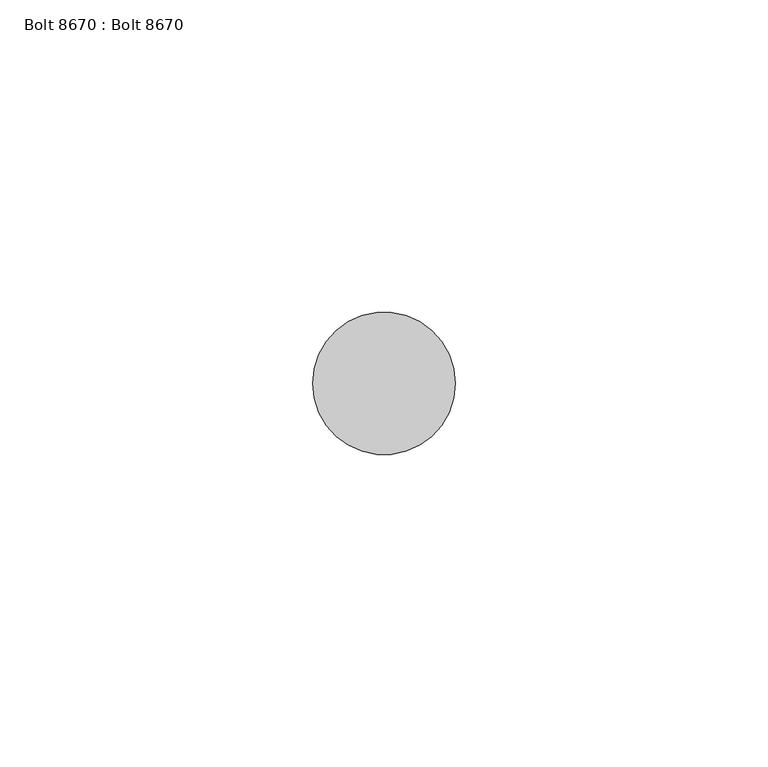
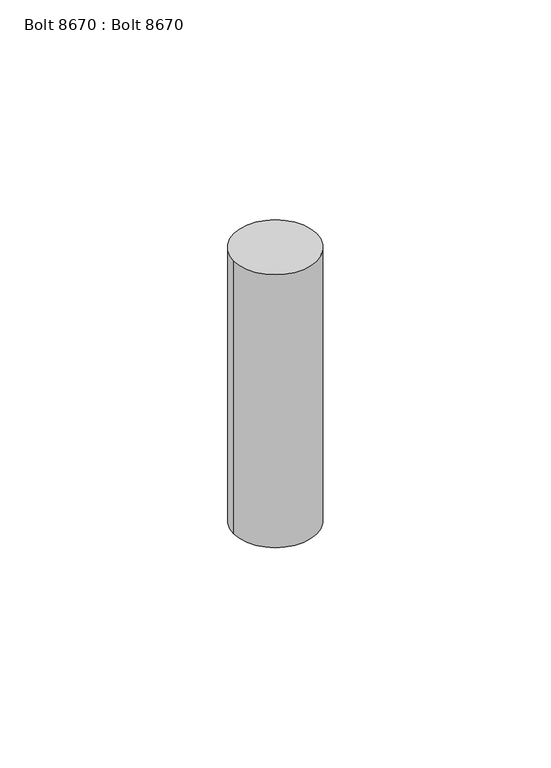
"""IFC4 building model written with IfcOpenShell, lengths in millimetres: proxy geometry, Bolt 8670 : Bolt 8670."""

from ifc_helpers import new_model, si_unit, point, frame, frame_2d, origin, place, context, project, spatial, circle_curve, trimmed, segment, composite_curve, outline, extrude, source, transform, mapped, element, save


def bolt_8670_bolt_8670_1f82a6c6(model_context):
    return source(origin(), model_context, "Body", "SweptSolid", [
        extrude(outline(composite_curve([segment(trimmed(circle_curve(frame_2d((7251.9702148, -1781.8449707)), 11.4045168), [point((7240.565698, -1781.8449707))], [point((7263.3747317, -1781.8449707))], False, "CARTESIAN"), True, "CONTINUOUS"), segment(trimmed(circle_curve(frame_2d((7251.9702148, -1781.8449707)), 11.4045168), [point((7263.3747317, -1781.8449707))], [point((7240.565698, -1781.8449707))], False, "CARTESIAN"), True, "CONTINUOUS")], self_intersect=False)), frame((0.0, 0.0, 40049.196), z_axis=(0.0, 0.0, 1.0), x_axis=(1.0, 0.0, 0.0)), (0.0, 0.0, 1.0), 79.375),
    ])


if __name__ == "__main__":
    model = new_model("IFC4")
    model_context = context("Model", 3, world=origin())
    ifc_project = project(units=[si_unit("LENGTHUNIT", "METRE", prefix="MILLI")], contexts=[model_context])
    site = spatial("IfcSite", under=ifc_project)
    building = spatial("IfcBuilding", under=site)
    placement = place(None, origin())
    bolt_8670_bolt_8670_shape = bolt_8670_bolt_8670_1f82a6c6(model_context)
    element("IfcBuildingElementProxy", 1, Name="Bolt 8670 : Bolt 8670", ObjectType="Bolt 8670 : Bolt 8670", at=placement, inside=building, context=model_context, shape_type="MappedRepresentation", body=[
        mapped(bolt_8670_bolt_8670_shape, transform((0.0, 0.0, 0.0), x_axis=(1.0, 0.0, 0.0), y_axis=(0.0, 1.0, 0.0), z_axis=(0.0, 0.0, 1.0))),
    ])
    save(model, "model.ifc")

# Revit data of these elements
# Type "Bolt 8670 : Bolt 8670"
#   NameOverride = "Bolt"
# Element 1 (IfcBuildingElementProxy, "Bolt 8670 : Bolt 8670")
#   Materials on its faces: "BOLTS CONCEALED BY FLOOR FINISH"
# Materials
#   "BOLTS CONCEALED BY FLOOR FINISH": class "Unassigned", colour RGB 128 128 128, transparency 0
